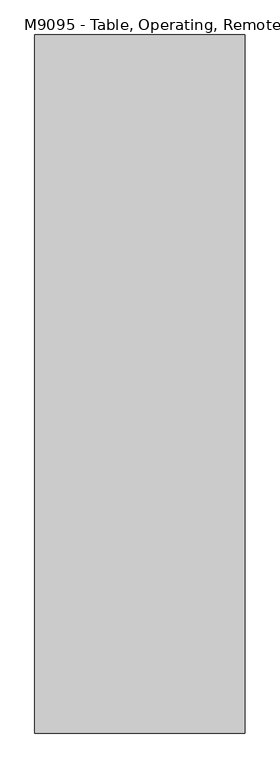
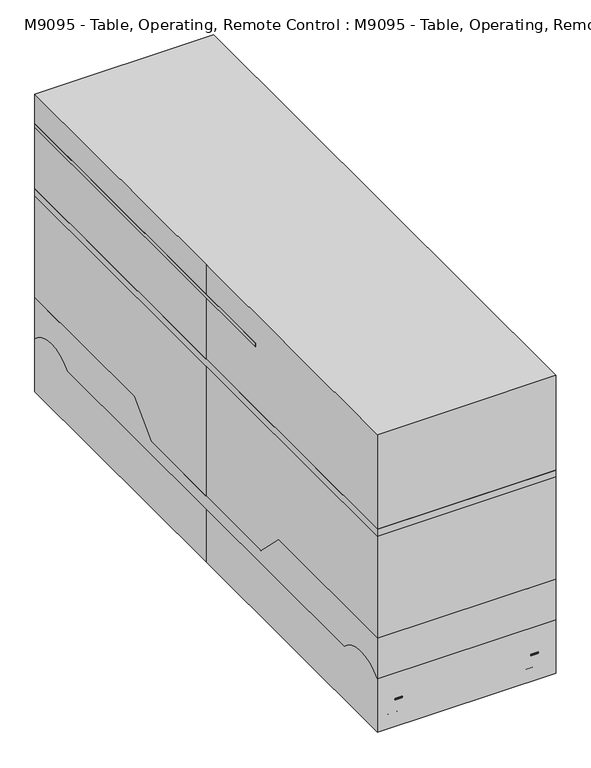
"""IFC4 building model written with IfcOpenShell, lengths in millimetres: proxy geometry, M9095 - Table, Operating, Remote Control : M9095 - Table, Operating, Remote Control."""

from ifc_helpers import new_model, si_unit, point, frame, frame_2d, origin, origin_with_axes, place, context, project, spatial, polyline, circle_curve, trimmed, segment, composite_curve, outline, extrude, source, transform, mapped, element, save


def m9095_table_operating_remote_control_m9095_table_operating_34d2ac3a(model_context):
    return source(origin(), model_context, "Body", "SweptSolid", [
        extrude(outline(composite_curve([segment(trimmed(circle_curve(frame_2d((-127.0, 647.7)), 63.5), [point((-63.5, 647.7))], [point((-190.5, 647.7))], False, "CARTESIAN"), True, "CONTINUOUS"), segment(trimmed(circle_curve(frame_2d((-127.0, 647.7)), 63.5), [point((-190.5, 647.7))], [point((-63.5, 647.7))], False, "CARTESIAN"), True, "CONTINUOUS")], self_intersect=False)), frame((0.0, 0.0, 428.573777), z_axis=(0.0, 0.0, 1.0), x_axis=(1.0, 0.0, 0.0)), (0.0, 0.0, 1.0), 304.8),
        extrude(outline(composite_curve([segment(trimmed(circle_curve(frame_2d((-127.0, 647.7)), 76.2), [point((-50.8, 647.7))], [point((-203.2, 647.7))], False, "CARTESIAN"), True, "CONTINUOUS"), segment(trimmed(circle_curve(frame_2d((-127.0, 647.7)), 76.2), [point((-203.2, 647.7))], [point((-50.8, 647.7))], False, "CARTESIAN"), True, "CONTINUOUS")], self_intersect=False)), frame((0.0, 0.0, 352.373777), z_axis=(0.0, 0.0, 1.0), x_axis=(1.0, 0.0, 0.0)), (0.0, 0.0, 1.0), 76.2),
        extrude(outline(composite_curve([segment(trimmed(circle_curve(frame_2d((-127.0, -647.7)), 63.5), [point((-63.5, -647.7))], [point((-190.5, -647.7))], False, "CARTESIAN"), True, "CONTINUOUS"), segment(trimmed(circle_curve(frame_2d((-127.0, -647.7)), 63.5), [point((-190.5, -647.7))], [point((-63.5, -647.7))], False, "CARTESIAN"), True, "CONTINUOUS")], self_intersect=False)), frame((0.0, 0.0, 428.573777), z_axis=(0.0, 0.0, 1.0), x_axis=(1.0, 0.0, 0.0)), (0.0, 0.0, 1.0), 304.8),
        extrude(outline(composite_curve([segment(trimmed(circle_curve(frame_2d((-127.0, -647.7)), 76.2), [point((-50.8, -647.7))], [point((-203.2, -647.7))], False, "CARTESIAN"), True, "CONTINUOUS"), segment(trimmed(circle_curve(frame_2d((-127.0, -647.7)), 76.2), [point((-203.2, -647.7))], [point((-50.8, -647.7))], False, "CARTESIAN"), True, "CONTINUOUS")], self_intersect=False)), frame((0.0, 0.0, 352.373777), z_axis=(0.0, 0.0, 1.0), x_axis=(1.0, 0.0, 0.0)), (0.0, 0.0, 1.0), 76.2),
        extrude(outline(composite_curve([segment(trimmed(circle_curve(frame_2d((127.0, 647.7)), 63.5), [point((63.5, 647.7))], [point((190.5, 647.7))], False, "CARTESIAN"), True, "CONTINUOUS"), segment(trimmed(circle_curve(frame_2d((127.0, 647.7)), 63.5), [point((190.5, 647.7))], [point((63.5, 647.7))], False, "CARTESIAN"), True, "CONTINUOUS")], self_intersect=False)), frame((0.0, 0.0, 428.573777), z_axis=(0.0, 0.0, 1.0), x_axis=(1.0, 0.0, 0.0)), (0.0, 0.0, 1.0), 304.8),
        extrude(outline(composite_curve([segment(trimmed(circle_curve(frame_2d((127.0, 647.7)), 76.2), [point((50.8, 647.7))], [point((203.2, 647.7))], False, "CARTESIAN"), True, "CONTINUOUS"), segment(trimmed(circle_curve(frame_2d((127.0, 647.7)), 76.2), [point((203.2, 647.7))], [point((50.8, 647.7))], False, "CARTESIAN"), True, "CONTINUOUS")], self_intersect=False)), frame((0.0, 0.0, 352.373777), z_axis=(0.0, 0.0, 1.0), x_axis=(1.0, 0.0, 0.0)), (0.0, 0.0, 1.0), 76.2),
        extrude(outline(composite_curve([segment(trimmed(circle_curve(frame_2d((127.0, -647.7)), 63.5), [point((63.5, -647.7))], [point((190.5, -647.7))], False, "CARTESIAN"), True, "CONTINUOUS"), segment(trimmed(circle_curve(frame_2d((127.0, -647.7)), 63.5), [point((190.5, -647.7))], [point((63.5, -647.7))], False, "CARTESIAN"), True, "CONTINUOUS")], self_intersect=False)), frame((0.0, 0.0, 428.573777), z_axis=(0.0, 0.0, 1.0), x_axis=(1.0, 0.0, 0.0)), (0.0, 0.0, 1.0), 304.8),
        extrude(outline(composite_curve([segment(trimmed(circle_curve(frame_2d((127.0, -647.7)), 76.2), [point((50.8, -647.7))], [point((203.2, -647.7))], False, "CARTESIAN"), True, "CONTINUOUS"), segment(trimmed(circle_curve(frame_2d((127.0, -647.7)), 76.2), [point((203.2, -647.7))], [point((50.8, -647.7))], False, "CARTESIAN"), True, "CONTINUOUS")], self_intersect=False)), frame((0.0, 0.0, 352.373777), z_axis=(0.0, 0.0, 1.0), x_axis=(1.0, 0.0, 0.0)), (0.0, 0.0, 1.0), 76.2),
        extrude(outline(polyline([(247.65, 146.05), (247.65, 317.5), (280.8025622, 317.5), (349.25, 184.15), (349.25, 146.05), (247.65, 146.05)])), frame((0.0, -127.0, 0.0), z_axis=(0.0, 1.0, 0.0), x_axis=(0.0, 0.0, 1.0)), (0.0, 0.0, 1.0), 254.0),
        extrude(outline(polyline([(0.0, -101.6), (0.0, 0.0), (76.2, 0.0), (76.2, -101.6), (0.0, -101.6)])), frame((295.5260184, 88.9, 292.0816229), z_axis=(0.45664846557060657, 0.0, 0.889647221595173), x_axis=(0.0, -1.0, 0.0)), (0.0, 0.0, 1.0), 12.7),
        extrude(outline(polyline([(0.0, -101.6), (0.0, 0.0), (76.2, 0.0), (76.2, -101.6), (0.0, -101.6)])), frame((205.1378607, -88.9, 338.477107), z_axis=(0.45664846557060657, 0.0, 0.889647221595173), x_axis=(0.0, 1.0, 0.0)), (0.0, 0.0, 1.0), 12.7),
        extrude(outline(polyline([(317.5, -304.8), (266.7, -304.8), (266.7, 1054.1), (317.5, 1054.1), (317.5, -304.8)])), frame((0.0, 0.0, 993.826223), z_axis=(0.0, 0.0, 1.0), x_axis=(1.0, 0.0, 0.0)), (0.0, 0.0, 1.0), 12.7),
        extrude(outline(polyline([(-266.7, -304.8), (-317.5, -304.8), (-317.5, 1054.1), (-266.7, 1054.1), (-266.7, -304.8)])), frame((0.0, 0.0, 993.826223), z_axis=(0.0, 0.0, 1.0), x_axis=(1.0, 0.0, 0.0)), (0.0, 0.0, 1.0), 12.7),
        extrude(outline(composite_curve([segment(trimmed(circle_curve(frame_2d((292.1, 952.5)), 19.05), [point((273.05, 952.5))], [point((311.15, 952.5))], False, "CARTESIAN"), True, "CONTINUOUS"), segment(trimmed(circle_curve(frame_2d((292.1, 952.5)), 19.05), [point((311.15, 952.5))], [point((273.05, 952.5))], False, "CARTESIAN"), True, "CONTINUOUS")], self_intersect=False)), frame((0.0, 0.0, 762.0), z_axis=(0.0, 0.0, 1.0), x_axis=(1.0, 0.0, 0.0)), (0.0, 0.0, 1.0), 231.826223),
        extrude(outline(composite_curve([segment(trimmed(circle_curve(frame_2d((292.1, 723.9)), 19.05), [point((273.05, 723.9))], [point((311.15, 723.9))], False, "CARTESIAN"), True, "CONTINUOUS"), segment(trimmed(circle_curve(frame_2d((292.1, 723.9)), 19.05), [point((311.15, 723.9))], [point((273.05, 723.9))], False, "CARTESIAN"), True, "CONTINUOUS")], self_intersect=False)), frame((0.0, 0.0, 762.0), z_axis=(0.0, 0.0, 1.0), x_axis=(1.0, 0.0, 0.0)), (0.0, 0.0, 1.0), 231.826223),
        extrude(outline(composite_curve([segment(trimmed(circle_curve(frame_2d((292.1, 495.3)), 19.05), [point((273.05, 495.3))], [point((311.15, 495.3))], False, "CARTESIAN"), True, "CONTINUOUS"), segment(trimmed(circle_curve(frame_2d((292.1, 495.3)), 19.05), [point((311.15, 495.3))], [point((273.05, 495.3))], False, "CARTESIAN"), True, "CONTINUOUS")], self_intersect=False)), frame((0.0, 0.0, 762.0), z_axis=(0.0, 0.0, 1.0), x_axis=(1.0, 0.0, 0.0)), (0.0, 0.0, 1.0), 231.826223),
        extrude(outline(composite_curve([segment(trimmed(circle_curve(frame_2d((292.1, 266.7)), 19.05), [point((273.05, 266.7))], [point((311.15, 266.7))], False, "CARTESIAN"), True, "CONTINUOUS"), segment(trimmed(circle_curve(frame_2d((292.1, 266.7)), 19.05), [point((311.15, 266.7))], [point((273.05, 266.7))], False, "CARTESIAN"), True, "CONTINUOUS")], self_intersect=False)), frame((0.0, 0.0, 762.0), z_axis=(0.0, 0.0, 1.0), x_axis=(1.0, 0.0, 0.0)), (0.0, 0.0, 1.0), 231.826223),
        extrude(outline(composite_curve([segment(trimmed(circle_curve(frame_2d((292.1, 38.1)), 19.05), [point((273.05, 38.1))], [point((311.15, 38.1))], False, "CARTESIAN"), True, "CONTINUOUS"), segment(trimmed(circle_curve(frame_2d((292.1, 38.1)), 19.05), [point((311.15, 38.1))], [point((273.05, 38.1))], False, "CARTESIAN"), True, "CONTINUOUS")], self_intersect=False)), frame((0.0, 0.0, 762.0), z_axis=(0.0, 0.0, 1.0), x_axis=(1.0, 0.0, 0.0)), (0.0, 0.0, 1.0), 231.826223),
        extrude(outline(composite_curve([segment(trimmed(circle_curve(frame_2d((292.1, -190.5)), 19.05), [point((273.05, -190.5))], [point((311.15, -190.5))], False, "CARTESIAN"), True, "CONTINUOUS"), segment(trimmed(circle_curve(frame_2d((292.1, -190.5)), 19.05), [point((311.15, -190.5))], [point((273.05, -190.5))], False, "CARTESIAN"), True, "CONTINUOUS")], self_intersect=False)), frame((0.0, 0.0, 762.0), z_axis=(0.0, 0.0, 1.0), x_axis=(1.0, 0.0, 0.0)), (0.0, 0.0, 1.0), 231.826223),
        extrude(outline(composite_curve([segment(trimmed(circle_curve(frame_2d((-292.1, 952.5)), 19.05), [point((-311.15, 952.5))], [point((-273.05, 952.5))], False, "CARTESIAN"), True, "CONTINUOUS"), segment(trimmed(circle_curve(frame_2d((-292.1, 952.5)), 19.05), [point((-273.05, 952.5))], [point((-311.15, 952.5))], False, "CARTESIAN"), True, "CONTINUOUS")], self_intersect=False)), frame((0.0, 0.0, 762.0), z_axis=(0.0, 0.0, 1.0), x_axis=(1.0, 0.0, 0.0)), (0.0, 0.0, 1.0), 231.826223),
        extrude(outline(composite_curve([segment(trimmed(circle_curve(frame_2d((-292.1, 723.9)), 19.05), [point((-311.15, 723.9))], [point((-273.05, 723.9))], False, "CARTESIAN"), True, "CONTINUOUS"), segment(trimmed(circle_curve(frame_2d((-292.1, 723.9)), 19.05), [point((-273.05, 723.9))], [point((-311.15, 723.9))], False, "CARTESIAN"), True, "CONTINUOUS")], self_intersect=False)), frame((0.0, 0.0, 762.0), z_axis=(0.0, 0.0, 1.0), x_axis=(1.0, 0.0, 0.0)), (0.0, 0.0, 1.0), 231.826223),
        extrude(outline(composite_curve([segment(trimmed(circle_curve(frame_2d((-292.1, 495.3)), 19.05), [point((-311.15, 495.3))], [point((-273.05, 495.3))], False, "CARTESIAN"), True, "CONTINUOUS"), segment(trimmed(circle_curve(frame_2d((-292.1, 495.3)), 19.05), [point((-273.05, 495.3))], [point((-311.15, 495.3))], False, "CARTESIAN"), True, "CONTINUOUS")], self_intersect=False)), frame((0.0, 0.0, 762.0), z_axis=(0.0, 0.0, 1.0), x_axis=(1.0, 0.0, 0.0)), (0.0, 0.0, 1.0), 231.826223),
        extrude(outline(composite_curve([segment(trimmed(circle_curve(frame_2d((-292.1, 266.7)), 19.05), [point((-311.15, 266.7))], [point((-273.05, 266.7))], False, "CARTESIAN"), True, "CONTINUOUS"), segment(trimmed(circle_curve(frame_2d((-292.1, 266.7)), 19.05), [point((-273.05, 266.7))], [point((-311.15, 266.7))], False, "CARTESIAN"), True, "CONTINUOUS")], self_intersect=False)), frame((0.0, 0.0, 762.0), z_axis=(0.0, 0.0, 1.0), x_axis=(1.0, 0.0, 0.0)), (0.0, 0.0, 1.0), 231.826223),
        extrude(outline(composite_curve([segment(trimmed(circle_curve(frame_2d((-292.1, 38.1)), 19.05), [point((-311.15, 38.1))], [point((-273.05, 38.1))], False, "CARTESIAN"), True, "CONTINUOUS"), segment(trimmed(circle_curve(frame_2d((-292.1, 38.1)), 19.05), [point((-273.05, 38.1))], [point((-311.15, 38.1))], False, "CARTESIAN"), True, "CONTINUOUS")], self_intersect=False)), frame((0.0, 0.0, 762.0), z_axis=(0.0, 0.0, 1.0), x_axis=(1.0, 0.0, 0.0)), (0.0, 0.0, 1.0), 231.826223),
        extrude(outline(composite_curve([segment(trimmed(circle_curve(frame_2d((-292.1, -190.5)), 19.05), [point((-311.15, -190.5))], [point((-273.05, -190.5))], False, "CARTESIAN"), True, "CONTINUOUS"), segment(trimmed(circle_curve(frame_2d((-292.1, -190.5)), 19.05), [point((-273.05, -190.5))], [point((-311.15, -190.5))], False, "CARTESIAN"), True, "CONTINUOUS")], self_intersect=False)), frame((0.0, 0.0, 762.0), z_axis=(0.0, 0.0, 1.0), x_axis=(1.0, 0.0, 0.0)), (0.0, 0.0, 1.0), 231.826223),
        extrude(outline(composite_curve([segment(polyline([(-215.9, 1028.7), (215.9, 1028.7)]), True, "CONTINUOUS"), segment(trimmed(circle_curve(frame_2d((215.9, 977.9)), 50.8), [point((215.9, 1028.7))], [point((266.7, 977.9))], False, "CARTESIAN"), True, "CONTINUOUS"), segment(polyline([(266.7, 977.9), (266.7, -977.9)]), True, "CONTINUOUS"), segment(trimmed(circle_curve(frame_2d((215.9, -977.9)), 50.8), [point((266.7, -977.9))], [point((215.9, -1028.7))], False, "CARTESIAN"), True, "CONTINUOUS"), segment(polyline([(215.9, -1028.7), (-215.9, -1028.7)]), True, "CONTINUOUS"), segment(trimmed(circle_curve(frame_2d((-215.9, -977.9)), 50.8), [point((-215.9, -1028.7))], [point((-266.7, -977.9))], False, "CARTESIAN"), True, "CONTINUOUS"), segment(polyline([(-266.7, -977.9), (-266.7, 977.9)]), True, "CONTINUOUS"), segment(trimmed(circle_curve(frame_2d((-215.9, 977.9)), 50.8), [point((-266.7, 977.9))], [point((-215.9, 1028.7))], False, "CARTESIAN"), True, "CONTINUOUS")], self_intersect=False)), frame((0.0, 0.0, 762.0), z_axis=(0.0, 0.0, 1.0), x_axis=(1.0, 0.0, 0.0)), (0.0, 0.0, 1.0), 50.8),
        extrude(outline(polyline([(317.5, 1054.1), (317.5, -1054.1), (-317.5, -1054.1), (-317.5, 1054.1), (317.5, 1054.1)])), frame((0.0, 0.0, 736.6), z_axis=(0.0, 0.0, 1.0), x_axis=(1.0, 0.0, 0.0)), (0.0, 0.0, 1.0), 25.4),
        extrude(outline(composite_curve([segment(trimmed(circle_curve(frame_2d((952.5, 101.6)), 101.6), [point((1054.1, 101.6))], [point((850.9, 101.6))], False, "CARTESIAN"), True, "CONTINUOUS"), segment(trimmed(circle_curve(frame_2d((952.5, 101.6)), 101.6), [point((850.9, 101.6))], [point((1054.1, 101.6))], False, "CARTESIAN"), True, "CONTINUOUS")], self_intersect=False)), frame((-254.0, 0.0, 0.0), z_axis=(1.0, 0.0, 0.0), x_axis=(0.0, 1.0, 0.0)), (0.0, 0.0, 1.0), 25.4),
        extrude(outline(composite_curve([segment(trimmed(circle_curve(frame_2d((-952.5, 101.6)), 101.6), [point((-1054.1, 101.6))], [point((-850.9, 101.6))], False, "CARTESIAN"), True, "CONTINUOUS"), segment(trimmed(circle_curve(frame_2d((-952.5, 101.6)), 101.6), [point((-850.9, 101.6))], [point((-1054.1, 101.6))], False, "CARTESIAN"), True, "CONTINUOUS")], self_intersect=False)), frame((-254.0, 0.0, 0.0), z_axis=(1.0, 0.0, 0.0), x_axis=(0.0, 1.0, 0.0)), (0.0, 0.0, 1.0), 25.4),
        extrude(outline(composite_curve([segment(trimmed(circle_curve(frame_2d((952.5, 101.6)), 101.6), [point((1054.1, 101.6))], [point((850.9, 101.6))], False, "CARTESIAN"), True, "CONTINUOUS"), segment(trimmed(circle_curve(frame_2d((952.5, 101.6)), 101.6), [point((850.9, 101.6))], [point((1054.1, 101.6))], False, "CARTESIAN"), True, "CONTINUOUS")], self_intersect=False)), frame((228.6, 0.0, 0.0), z_axis=(1.0, 0.0, 0.0), x_axis=(0.0, 1.0, 0.0)), (0.0, 0.0, 1.0), 25.4),
        extrude(outline(composite_curve([segment(trimmed(circle_curve(frame_2d((-952.5, 98.373777)), 101.6), [point((-1054.1, 98.373777))], [point((-850.9, 98.373777))], False, "CARTESIAN"), True, "CONTINUOUS"), segment(trimmed(circle_curve(frame_2d((-952.5, 98.373777)), 101.6), [point((-850.9, 98.373777))], [point((-1054.1, 98.373777))], False, "CARTESIAN"), True, "CONTINUOUS")], self_intersect=False)), frame((228.6, 0.0, 0.0), z_axis=(1.0, 0.0, 0.0), x_axis=(0.0, 1.0, 0.0)), (0.0, 0.0, 1.0), 25.4),
        extrude(outline(composite_curve([segment(trimmed(circle_curve(frame_2d((241.3, 952.5)), 25.4), [point((215.9, 952.5))], [point((266.7, 952.5))], False, "CARTESIAN"), True, "CONTINUOUS"), segment(trimmed(circle_curve(frame_2d((241.3, 952.5)), 25.4), [point((266.7, 952.5))], [point((215.9, 952.5))], False, "CARTESIAN"), True, "CONTINUOUS")], self_intersect=False)), frame((0.0, 0.0, 222.25), z_axis=(0.0, 0.0, 1.0), x_axis=(1.0, 0.0, 0.0)), (0.0, 0.0, 1.0), 25.4),
        extrude(outline(polyline([(215.9, 990.6), (266.7, 990.6), (266.7, 914.4), (215.9, 914.4), (215.9, 990.6)])), frame((0.0, 0.0, 209.55), z_axis=(0.0, 0.0, 1.0), x_axis=(1.0, 0.0, 0.0)), (0.0, 0.0, 1.0), 12.7),
        extrude(outline(polyline([(254.0, 965.2), (266.7, 965.2), (266.7, 939.8), (254.0, 939.8), (254.0, 965.2)])), frame((0.0, 0.0, 101.6), z_axis=(0.0, 0.0, 1.0), x_axis=(1.0, 0.0, 0.0)), (0.0, 0.0, 1.0), 107.95),
        extrude(outline(polyline([(215.9, 965.2), (228.6, 965.2), (228.6, 939.8), (215.9, 939.8), (215.9, 965.2)])), frame((0.0, 0.0, 101.6), z_axis=(0.0, 0.0, 1.0), x_axis=(1.0, 0.0, 0.0)), (0.0, 0.0, 1.0), 107.95),
        extrude(outline(composite_curve([segment(trimmed(circle_curve(frame_2d((241.3, -952.5)), 25.4), [point((215.9, -952.5))], [point((266.7, -952.5))], False, "CARTESIAN"), True, "CONTINUOUS"), segment(trimmed(circle_curve(frame_2d((241.3, -952.5)), 25.4), [point((266.7, -952.5))], [point((215.9, -952.5))], False, "CARTESIAN"), True, "CONTINUOUS")], self_intersect=False)), frame((0.0, 0.0, 222.25), z_axis=(0.0, 0.0, 1.0), x_axis=(1.0, 0.0, 0.0)), (0.0, 0.0, 1.0), 25.4),
        extrude(outline(polyline([(266.7, -990.6), (215.9, -990.6), (215.9, -914.4), (266.7, -914.4), (266.7, -990.6)])), frame((0.0, 0.0, 209.55), z_axis=(0.0, 0.0, 1.0), x_axis=(1.0, 0.0, 0.0)), (0.0, 0.0, 1.0), 12.7),
        extrude(outline(polyline([(228.6, -965.2), (215.9, -965.2), (215.9, -939.8), (228.6, -939.8), (228.6, -965.2)])), frame((0.0, 0.0, 101.6), z_axis=(0.0, 0.0, 1.0), x_axis=(1.0, 0.0, 0.0)), (0.0, 0.0, 1.0), 107.95),
        extrude(outline(polyline([(266.7, -965.2), (254.0, -965.2), (254.0, -939.8), (266.7, -939.8), (266.7, -965.2)])), frame((0.0, 0.0, 101.6), z_axis=(0.0, 0.0, 1.0), x_axis=(1.0, 0.0, 0.0)), (0.0, 0.0, 1.0), 107.95),
        extrude(outline(composite_curve([segment(trimmed(circle_curve(frame_2d((-241.3, 952.5)), 25.4), [point((-215.9, 952.5))], [point((-266.7, 952.5))], False, "CARTESIAN"), True, "CONTINUOUS"), segment(trimmed(circle_curve(frame_2d((-241.3, 952.5)), 25.4), [point((-266.7, 952.5))], [point((-215.9, 952.5))], False, "CARTESIAN"), True, "CONTINUOUS")], self_intersect=False)), frame((0.0, 0.0, 222.25), z_axis=(0.0, 0.0, 1.0), x_axis=(1.0, 0.0, 0.0)), (0.0, 0.0, 1.0), 25.4),
        extrude(outline(polyline([(-266.7, 990.6), (-215.9, 990.6), (-215.9, 914.4), (-266.7, 914.4), (-266.7, 990.6)])), frame((0.0, 0.0, 209.55), z_axis=(0.0, 0.0, 1.0), x_axis=(1.0, 0.0, 0.0)), (0.0, 0.0, 1.0), 12.7),
        extrude(outline(polyline([(-228.6, 965.2), (-215.9, 965.2), (-215.9, 939.8), (-228.6, 939.8), (-228.6, 965.2)])), frame((0.0, 0.0, 101.6), z_axis=(0.0, 0.0, 1.0), x_axis=(1.0, 0.0, 0.0)), (0.0, 0.0, 1.0), 107.95),
        extrude(outline(polyline([(-266.7, 965.2), (-254.0, 965.2), (-254.0, 939.8), (-266.7, 939.8), (-266.7, 965.2)])), frame((0.0, 0.0, 101.6), z_axis=(0.0, 0.0, 1.0), x_axis=(1.0, 0.0, 0.0)), (0.0, 0.0, 1.0), 107.95),
        extrude(outline(composite_curve([segment(trimmed(circle_curve(frame_2d((-241.3, -952.5)), 25.4), [point((-215.9, -952.5))], [point((-266.7, -952.5))], False, "CARTESIAN"), True, "CONTINUOUS"), segment(trimmed(circle_curve(frame_2d((-241.3, -952.5)), 25.4), [point((-266.7, -952.5))], [point((-215.9, -952.5))], False, "CARTESIAN"), True, "CONTINUOUS")], self_intersect=False)), frame((0.0, 0.0, 222.25), z_axis=(0.0, 0.0, 1.0), x_axis=(1.0, 0.0, 0.0)), (0.0, 0.0, 1.0), 25.4),
        extrude(outline(polyline([(-215.9, -990.6), (-266.7, -990.6), (-266.7, -914.4), (-215.9, -914.4), (-215.9, -990.6)])), frame((0.0, 0.0, 209.55), z_axis=(0.0, 0.0, 1.0), x_axis=(1.0, 0.0, 0.0)), (0.0, 0.0, 1.0), 12.7),
        extrude(outline(polyline([(-254.0, -965.2), (-266.7, -965.2), (-266.7, -939.8), (-254.0, -939.8), (-254.0, -965.2)])), frame((0.0, 0.0, 101.6), z_axis=(0.0, 0.0, 1.0), x_axis=(1.0, 0.0, 0.0)), (0.0, 0.0, 1.0), 107.95),
        extrude(outline(polyline([(-215.9, -965.2), (-228.6, -965.2), (-228.6, -939.8), (-215.9, -939.8), (-215.9, -965.2)])), frame((0.0, 0.0, 101.6), z_axis=(0.0, 0.0, 1.0), x_axis=(1.0, 0.0, 0.0)), (0.0, 0.0, 1.0), 107.95),
        extrude(outline(composite_curve([segment(polyline([(-1054.1, 352.373777), (-444.5, 352.373777), (-339.776223, 247.65), (339.776223, 247.65), (444.5, 352.373777), (1054.1, 352.373777), (1054.1, 199.973777)]), True, "CONTINUOUS"), segment(trimmed(circle_curve(frame_2d((952.5, 101.6)), 141.4212148), [point((1054.1, 199.973777))], [point((850.9, 199.973777))], True, "CARTESIAN"), True, "CONTINUOUS"), segment(polyline([(850.9, 199.973777), (-850.9, 199.973777)]), True, "CONTINUOUS"), segment(trimmed(circle_curve(frame_2d((-952.5, 101.6)), 141.4212148), [point((-850.9, 199.973777))], [point((-1054.1, 199.973777))], True, "CARTESIAN"), True, "CONTINUOUS"), segment(polyline([(-1054.1, 199.973777), (-1054.1, 352.373777)]), True, "CONTINUOUS")], self_intersect=False)), frame((-317.5, 0.0, 0.0), z_axis=(1.0, 0.0, 0.0), x_axis=(0.0, 1.0, 0.0)), (0.0, 0.0, 1.0), 635.0),
        extrude(outline(polyline([(-317.5, 1054.1), (317.5, 1054.1), (317.5, -1054.1), (-317.5, -1054.1), (-317.5, 0.0), (-317.5, 1054.1)])), origin_with_axes(), (0.0, 0.0, 1.0), 1117.6),
    ])


if __name__ == "__main__":
    model = new_model("IFC4")
    model_context = context("Model", 3, world=origin())
    ifc_project = project(units=[si_unit("LENGTHUNIT", "METRE", prefix="MILLI")], contexts=[model_context])
    site = spatial("IfcSite", under=ifc_project)
    building = spatial("IfcBuilding", under=site)
    placement = place(None, origin())
    m9095_table_operating_remote_control_m9095_table_operating_shape = m9095_table_operating_remote_control_m9095_table_operating_34d2ac3a(model_context)
    element("IfcBuildingElementProxy", 1, Name="M9095 - Table, Operating, Remote Control : M9095 - Table, Operating, Remote Control", ObjectType="M9095 - Table, Operating, Remote Control : M9095 - Table, Operating, Remote Control", at=placement, inside=building, context=model_context, shape_type="MappedRepresentation", body=[
        mapped(m9095_table_operating_remote_control_m9095_table_operating_shape, transform((0.0, 0.0, 0.0), x_axis=(1.0, 0.0, 0.0), y_axis=(0.0, 1.0, 0.0), z_axis=(0.0, 0.0, 1.0))),
    ])
    save(model, "model.ifc")

# Revit data of these elements
# Project information
#   Room Abbreviation = "LDDR1"
#   Room Description = "Operating Room, Labor & Delivery, C-Section (LDDR1)"
#   Sheets - Total = "6"
#   Project Issue Date = "Issue Date"
#   Project Status = "Project Status"
#   Client Name = "Owner"
#   Project Address = "Enter address here"
#   Project Name = "Project Name"
#   Project Number = "Project Number"
#   Publication Date = "30-Jan-15"
# Type "M9095 - Table, Operating, Remote Control : M9095 - Table, Operating, Remote Control"
#   Watts2 = "0"
#   Watts1 = "600"
#   Unit_Issue = "EA"
#   UTIL_6_Misc = "-"
#   UTIL_5_NonMedGas = "-"
#   UTIL_4_MiscGas = "-"
#   UTIL_3_MedGas = "-"
#   UTIL_2_Elec = "A"
#   UTIL_1_WaterDrain = "-"
#   Nomenclature = "Table, Operating, Remote Control"
#   NSN = "6530"
#   Location [instance default] = ""
#   JSN = "M9095"
#   Fund_Source_VA = "-"
#   Fund_Source_Navy = "-"
#   Fund_Source_Army = "-"
#   Fund_Source_AF = "-"
#   ELEC_Volts2 = "0"
#   ELEC_Volts1 = "120"
#   ELEC_Phase2 = "0"
#   ELEC_Phase1 = "1"
#   ELEC_HertzSwitch = "0"
#   ELEC_HertzDependent = "-1"
#   ELEC_Hertz = "60"
#   ELEC_Amps2 = "0"
#   ELEC_Amps1 = "5"
#   DetailDescription = "Remote control surgical table. Table is a stainless steel pedestal type mounted on conductive locking casters. It consists of an Electro-hydraulic system with remote control and foot pedals. Unit's positioning capabilities include lateral tilt of 30 degrees, Trendelenburg and reverse Trendelenburg. It is equipped with side rails, kidney bridge and a radio translucent top. Table is designed for a variety of procedures in the operating room."
#   CAT_VA = "C"
#   CAT_Navy = "C"
#   CAT_IHS = "-"
#   CAT_Army = "C"
#   CAT_AF = "C"
#   BTUperhour = "0"
#   Weight_IP = 750
#   DIM_Width_IP = 2' - 1"
#   DIM_Height_IP = 3' - 8"
#   DIM_Depth_IP = 6' - 11"
# Element 1 (IfcBuildingElementProxy, "M9095 - Table, Operating, Remote Control : M9095 - Table, Operating, Remote Control")
#   Materials on its faces: "EquipSpace"
# Materials
#   "EquipSpace": class "Unassigned", colour RGB 221 217 195, transparency 0.5
